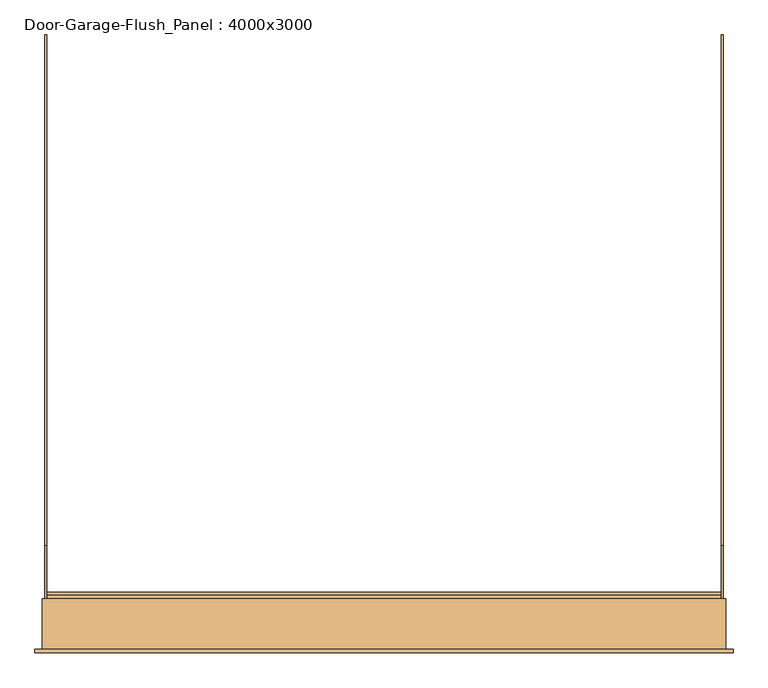
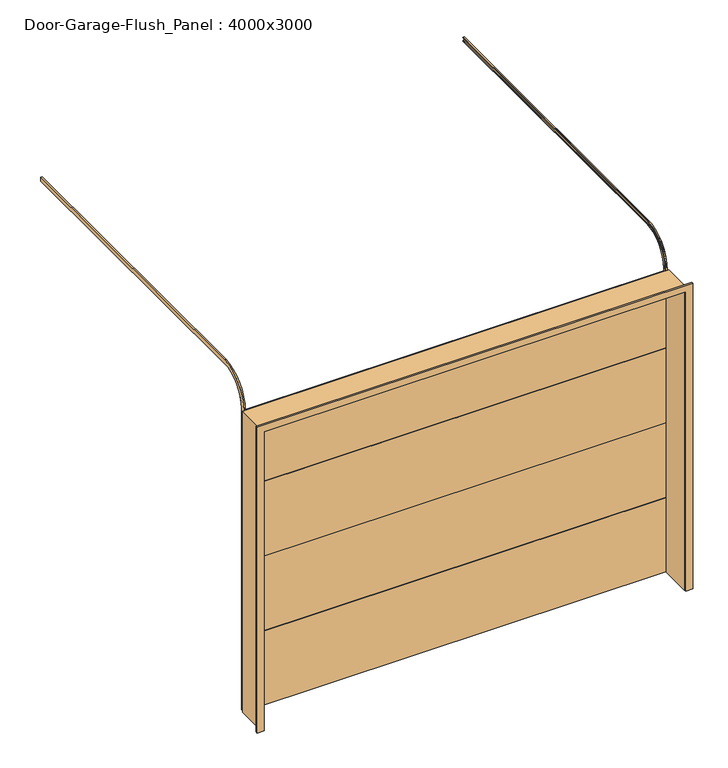
"""IFC4 building model written with IfcOpenShell, lengths in millimetres: door geometry, Door-Garage-Flush_Panel : 4000x3000."""

from ifc_helpers import new_model, si_unit, frame, origin, place, context, project, spatial, polyline, circle_curve, outline, extrude, source, transform, mapped, element, save
from ifc_brep_helpers import plane_surface, cylinder_surface, revolved_surface, advanced_brep


def door_garage_flush_panel_4000x3000_59d66c1f(model_context):
    return source(origin(), model_context, "Body", "SolidModel", [
        extrude(outline(polyline([(175.4, 3003.175), (191.275, 3003.175), (191.275, 2256.35), (169.05, 2256.35), (169.05, 2250.0), (153.175, 2250.0), (153.175, 2996.825), (175.4, 2996.825), (175.4, 3003.175)])), frame((-2000.0, 0.0, 0.0), z_axis=(1.0, 0.0, 0.0), x_axis=(0.0, 1.0, 0.0)), (0.0, 0.0, 1.0), 4000.0),
        extrude(outline(polyline([(175.4, 2253.175), (191.275, 2253.175), (191.275, 1506.35), (169.05, 1506.35), (169.05, 1500.0), (153.175, 1500.0), (153.175, 2246.825), (175.4, 2246.825), (175.4, 2253.175)])), frame((-2000.0, 0.0, 0.0), z_axis=(1.0, 0.0, 0.0), x_axis=(0.0, 1.0, 0.0)), (0.0, 0.0, 1.0), 4000.0),
        extrude(outline(polyline([(175.4, 1503.175), (191.275, 1503.175), (191.275, 756.35), (169.05, 756.35), (169.05, 750.0), (153.175, 750.0), (153.175, 1496.825), (175.4, 1496.825), (175.4, 1503.175)])), frame((-2000.0, 0.0, 0.0), z_axis=(1.0, 0.0, 0.0), x_axis=(0.0, 1.0, 0.0)), (0.0, 0.0, 1.0), 4000.0),
        extrude(outline(polyline([(175.4, 753.175), (191.275, 753.175), (191.275, 6.35), (169.05, 6.35), (169.05, 0.0), (153.175, 0.0), (153.175, 746.825), (175.4, 746.825), (175.4, 753.175)])), frame((-2000.0, 0.0, 0.0), z_axis=(1.0, 0.0, 0.0), x_axis=(0.0, 1.0, 0.0)), (0.0, 0.0, 1.0), 4000.0),
        extrude(outline(polyline([(0.0, 2025.4), (3025.4, 2025.4), (3025.4, -2025.4), (0.0, -2025.4), (0.0, -2000.0), (3000.0, -2000.0), (3000.0, 2000.0), (0.0, 2000.0), (0.0, 2025.4)])), frame((0.0, -146.825, 0.0), z_axis=(0.0, 1.0, 0.0), x_axis=(0.0, 0.0, 1.0)), (0.0, 0.0, 1.0), 300.0),
        advanced_brep(
        [(2012.7, 3496.075, 3304.8), (2000.0, 3496.075, 3304.8), (2000.0, 3496.075, 3307.975), (2009.525, 3496.075, 3307.975), (2009.525, 3496.075, 3339.725), (2000.0, 3496.075, 3339.725), (2000.0, 3496.075, 3342.9), (2012.7, 3496.075, 3342.9), (2012.7, 470.675, 3342.9), (2012.7, 153.175, 3025.4), (2012.7, 153.175, 0.0), (2012.7, 191.275, 0.0), (2012.7, 191.275, 3025.4), (2012.7, 470.675, 3304.8), (2000.0, 470.675, 3342.9), (2000.0, 470.675, 3339.725), (2000.0, 156.35, 3025.4), (2000.0, 156.35, 0.0), (2000.0, 153.175, 0.0), (2000.0, 153.175, 3025.4), (2009.525, 470.675, 3339.725), (2009.525, 470.675, 3307.975), (2009.525, 188.1, 3025.4), (2009.525, 188.1, 0.0), (2009.525, 156.35, 0.0), (2009.525, 156.35, 3025.4), (2000.0, 470.675, 3307.975), (2000.0, 470.675, 3304.8), (2000.0, 191.275, 3025.4), (2000.0, 191.275, 0.0), (2000.0, 188.1, 0.0), (2000.0, 188.1, 3025.4)],
        [
            (0, 1),
            (1, 2),
            (2, 3),
            (3, 4),
            (4, 5),
            (5, 6),
            (6, 7),
            (7, 0),
            (7, 8),
            (8, 9, circle_curve(frame((2012.7, 470.675, 3025.4), z_axis=(1.0, 0.0, 0.0), x_axis=(0.0, 0.0, 1.0)), 317.5)),
            (9, 10),
            (10, 11),
            (11, 12),
            (12, 13, circle_curve(frame((2012.7, 470.675, 3025.4), z_axis=(-1.0, 0.0, 0.0), x_axis=(0.0, 0.0, 1.0)), 279.4)),
            (13, 0),
            (6, 14),
            (14, 8),
            (5, 15),
            (15, 16, circle_curve(frame((2000.0, 470.675, 3025.4), z_axis=(1.0, 0.0, 0.0), x_axis=(0.0, 0.0, 1.0)), 314.325)),
            (16, 17),
            (17, 18),
            (18, 19),
            (19, 14, circle_curve(frame((2000.0, 470.675, 3025.4), z_axis=(-1.0, 0.0, 0.0), x_axis=(0.0, 0.0, 1.0)), 317.5)),
            (4, 20),
            (20, 15),
            (3, 21),
            (21, 22, circle_curve(frame((2009.525, 470.675, 3025.4), z_axis=(1.0, 0.0, 0.0), x_axis=(0.0, 0.0, 1.0)), 282.575)),
            (22, 23),
            (23, 24),
            (24, 25),
            (25, 20, circle_curve(frame((2009.525, 470.675, 3025.4), z_axis=(-1.0, 0.0, 0.0), x_axis=(0.0, 0.0, 1.0)), 314.325)),
            (2, 26),
            (26, 21),
            (1, 27),
            (27, 28, circle_curve(frame((2000.0, 470.675, 3025.4), z_axis=(1.0, 0.0, 0.0), x_axis=(0.0, 0.0, 1.0)), 279.4)),
            (28, 29),
            (29, 30),
            (30, 31),
            (31, 26, circle_curve(frame((2000.0, 470.675, 3025.4), z_axis=(-1.0, 0.0, 0.0), x_axis=(0.0, 0.0, 1.0)), 282.575)),
            (13, 27),
            (19, 9),
            (25, 16),
            (31, 22),
            (12, 28),
            (10, 18),
            (17, 24),
            (23, 30),
            (29, 11),
        ],
        [
            plane_surface(frame((0.0, 3496.075, 3304.8), z_axis=(0.0, 1.0, 0.0), x_axis=(1.0, 0.0, 0.0))),
            plane_surface(frame((2012.7, 3496.075, 3304.8), z_axis=(1.0, 0.0, 0.0), x_axis=(0.0, -1.0, 0.0))),
            plane_surface(frame((2012.7, 3496.075, 3342.9), z_axis=(0.0, 0.0, 1.0), x_axis=(0.0, -1.0, 0.0))),
            plane_surface(frame((2000.0, 3496.075, 3342.9), z_axis=(-1.0, 0.0, 0.0), x_axis=(0.0, -1.0, 0.0))),
            plane_surface(frame((2000.0, 3496.075, 3339.725), z_axis=(0.0, 0.0, -1.0), x_axis=(0.0, -1.0, 0.0))),
            plane_surface(frame((2009.525, 3496.075, 3339.725), z_axis=(-1.0, 0.0, 0.0), x_axis=(0.0, -1.0, 0.0))),
            plane_surface(frame((2009.525, 3496.075, 3307.975), z_axis=(0.0, 0.0, 1.0), x_axis=(0.0, -1.0, 0.0))),
            plane_surface(frame((2000.0, 3496.075, 3307.975), z_axis=(-1.0, 0.0, 0.0), x_axis=(0.0, -1.0, 0.0))),
            plane_surface(frame((2000.0, 3496.075, 3304.8), z_axis=(0.0, 0.0, -1.0), x_axis=(0.0, -1.0, 0.0))),
            cylinder_surface(frame((0.0, 470.675, 3025.4), z_axis=(-1.0, 0.0, 0.0), x_axis=(0.0, 0.0, 1.0)), 317.5),
            revolved_surface(polyline([(2000.0, 470.675, 3339.725), (2009.525, 470.675, 3339.725)]), (0.0, 470.675, 3025.4), (-1.0, 0.0, 0.0)),
            cylinder_surface(frame((0.0, 470.675, 3025.4), z_axis=(-1.0, 0.0, 0.0), x_axis=(0.0, 0.0, 1.0)), 282.575),
            revolved_surface(polyline([(2000.0, 470.675, 3304.8), (2012.7, 470.675, 3304.8)]), (0.0, 470.675, 3025.4), (-1.0, 0.0, 0.0)),
            plane_surface(frame((0.0, 191.275, 0.0), z_axis=(0.0, 0.0, -1.0), x_axis=(1.0, 0.0, 0.0))),
            plane_surface(frame((2012.7, 153.175, 3025.4), z_axis=(0.0, -1.0, 0.0), x_axis=(0.0, 0.0, -1.0))),
            plane_surface(frame((2000.0, 156.35, 3025.4), z_axis=(0.0, 1.0, 0.0), x_axis=(0.0, 0.0, -1.0))),
            plane_surface(frame((2009.525, 188.1, 3025.4), z_axis=(0.0, -1.0, 0.0), x_axis=(0.0, 0.0, -1.0))),
            plane_surface(frame((2000.0, 191.275, 3025.4), z_axis=(0.0, 1.0, 0.0), x_axis=(0.0, 0.0, -1.0))),
        ],
        [
            (0, [[1, 2, 3, 4, 5, 6, 7, 8]]),
            (1, [[9, 10, 11, 12, 13, 14, 15, -8]]),
            (2, [[16, 17, -9, -7]]),
            (3, [[18, 19, 20, 21, 22, 23, -16, -6]]),
            (4, [[24, 25, -18, -5]]),
            (5, [[26, 27, 28, 29, 30, 31, -24, -4]]),
            (6, [[32, 33, -26, -3]]),
            (7, [[34, 35, 36, 37, 38, 39, -32, -2]]),
            (8, [[-15, 40, -34, -1]]),
            (9, [[41, -10, -17, -23]]),
            (10, [[42, -19, -25, -31]]),
            (11, [[43, -27, -33, -39]]),
            (12, [[44, -35, -40, -14]]),
            (13, [[-12, 45, -21, 46, -29, 47, -37, 48]]),
            (14, [[-22, -45, -11, -41]]),
            (15, [[-30, -46, -20, -42]]),
            (16, [[-38, -47, -28, -43]]),
            (17, [[-13, -48, -36, -44]]),
        ],
    ),
        advanced_brep(
        [(-2012.7, 3496.075, 3304.8), (-2012.7, 3496.075, 3342.9), (-2000.0, 3496.075, 3342.9), (-2000.0, 3496.075, 3339.725), (-2009.525, 3496.075, 3339.725), (-2009.525, 3496.075, 3307.975), (-2000.0, 3496.075, 3307.975), (-2000.0, 3496.075, 3304.8), (-2000.0, 470.675, 3304.8), (-2012.7, 470.675, 3304.8), (-2000.0, 470.675, 3307.975), (-2000.0, 188.1, 3025.4), (-2000.0, 188.1, 0.0), (-2000.0, 191.275, 0.0), (-2000.0, 191.275, 3025.4), (-2009.525, 470.675, 3307.975), (-2009.525, 470.675, 3339.725), (-2009.525, 156.35, 3025.4), (-2009.525, 156.35, 0.0), (-2009.525, 188.1, 0.0), (-2009.525, 188.1, 3025.4), (-2000.0, 470.675, 3339.725), (-2000.0, 470.675, 3342.9), (-2000.0, 153.175, 3025.4), (-2000.0, 153.175, 0.0), (-2000.0, 156.35, 0.0), (-2000.0, 156.35, 3025.4), (-2012.7, 470.675, 3342.9), (-2012.7, 191.275, 3025.4), (-2012.7, 191.275, 0.0), (-2012.7, 153.175, 0.0), (-2012.7, 153.175, 3025.4)],
        [
            (0, 1),
            (1, 2),
            (2, 3),
            (3, 4),
            (4, 5),
            (5, 6),
            (6, 7),
            (7, 0),
            (7, 8),
            (8, 9),
            (9, 0),
            (6, 10),
            (10, 11, circle_curve(frame((-2000.0, 470.675, 3025.4), z_axis=(1.0, 0.0, 0.0), x_axis=(0.0, 0.0, 1.0)), 282.575)),
            (11, 12),
            (12, 13),
            (13, 14),
            (14, 8, circle_curve(frame((-2000.0, 470.675, 3025.4), z_axis=(-1.0, 0.0, 0.0), x_axis=(0.0, 0.0, 1.0)), 279.4)),
            (5, 15),
            (15, 10),
            (4, 16),
            (16, 17, circle_curve(frame((-2009.525, 470.675, 3025.4), z_axis=(1.0, 0.0, 0.0), x_axis=(0.0, 0.0, 1.0)), 314.325)),
            (17, 18),
            (18, 19),
            (19, 20),
            (20, 15, circle_curve(frame((-2009.525, 470.675, 3025.4), z_axis=(-1.0, 0.0, 0.0), x_axis=(0.0, 0.0, 1.0)), 282.575)),
            (3, 21),
            (21, 16),
            (2, 22),
            (22, 23, circle_curve(frame((-2000.0, 470.675, 3025.4), z_axis=(1.0, 0.0, 0.0), x_axis=(0.0, 0.0, 1.0)), 317.5)),
            (23, 24),
            (24, 25),
            (25, 26),
            (26, 21, circle_curve(frame((-2000.0, 470.675, 3025.4), z_axis=(-1.0, 0.0, 0.0), x_axis=(0.0, 0.0, 1.0)), 314.325)),
            (1, 27),
            (27, 22),
            (9, 28, circle_curve(frame((-2012.7, 470.675, 3025.4), z_axis=(1.0, 0.0, 0.0), x_axis=(0.0, 0.0, 1.0)), 279.4)),
            (28, 29),
            (29, 30),
            (30, 31),
            (31, 27, circle_curve(frame((-2012.7, 470.675, 3025.4), z_axis=(-1.0, 0.0, 0.0), x_axis=(0.0, 0.0, 1.0)), 317.5)),
            (14, 28),
            (20, 11),
            (26, 17),
            (31, 23),
            (29, 13),
            (12, 19),
            (18, 25),
            (24, 30),
        ],
        [
            plane_surface(frame((0.0, 3496.075, 3304.8), z_axis=(0.0, 1.0, 0.0), x_axis=(1.0, 0.0, 0.0))),
            plane_surface(frame((-2012.7, 3496.075, 3304.8), z_axis=(0.0, 0.0, -1.0), x_axis=(0.0, -1.0, 0.0))),
            plane_surface(frame((-2000.0, 3496.075, 3304.8), z_axis=(1.0, 0.0, 0.0), x_axis=(0.0, -1.0, 0.0))),
            plane_surface(frame((-2000.0, 3496.075, 3307.975), z_axis=(0.0, 0.0, 1.0), x_axis=(0.0, -1.0, 0.0))),
            plane_surface(frame((-2009.525, 3496.075, 3307.975), z_axis=(1.0, 0.0, 0.0), x_axis=(0.0, -1.0, 0.0))),
            plane_surface(frame((-2009.525, 3496.075, 3339.725), z_axis=(0.0, 0.0, -1.0), x_axis=(0.0, -1.0, 0.0))),
            plane_surface(frame((-2000.0, 3496.075, 3339.725), z_axis=(1.0, 0.0, 0.0), x_axis=(0.0, -1.0, 0.0))),
            plane_surface(frame((-2000.0, 3496.075, 3342.9), z_axis=(0.0, 0.0, 1.0), x_axis=(0.0, -1.0, 0.0))),
            plane_surface(frame((-2012.7, 3496.075, 3342.9), z_axis=(-1.0, 0.0, 0.0), x_axis=(0.0, -1.0, 0.0))),
            revolved_surface(polyline([(-2012.7, 470.675, 3304.8), (-2000.0, 470.675, 3304.8)]), (0.0, 470.675, 3025.4), (-1.0, 0.0, 0.0)),
            cylinder_surface(frame((0.0, 470.675, 3025.4), z_axis=(-1.0, 0.0, 0.0), x_axis=(0.0, 0.0, 1.0)), 282.575),
            revolved_surface(polyline([(-2009.525, 470.675, 3339.725), (-2000.0, 470.675, 3339.725)]), (0.0, 470.675, 3025.4), (-1.0, 0.0, 0.0)),
            cylinder_surface(frame((0.0, 470.675, 3025.4), z_axis=(-1.0, 0.0, 0.0), x_axis=(0.0, 0.0, 1.0)), 317.5),
            plane_surface(frame((0.0, 191.275, 0.0), z_axis=(0.0, 0.0, -1.0), x_axis=(1.0, 0.0, 0.0))),
            plane_surface(frame((-2012.7, 191.275, 3025.4), z_axis=(0.0, 1.0, 0.0), x_axis=(0.0, 0.0, -1.0))),
            plane_surface(frame((-2000.0, 188.1, 3025.4), z_axis=(0.0, -1.0, 0.0), x_axis=(0.0, 0.0, -1.0))),
            plane_surface(frame((-2009.525, 156.35, 3025.4), z_axis=(0.0, 1.0, 0.0), x_axis=(0.0, 0.0, -1.0))),
            plane_surface(frame((-2000.0, 153.175, 3025.4), z_axis=(0.0, -1.0, 0.0), x_axis=(0.0, 0.0, -1.0))),
        ],
        [
            (0, [[1, 2, 3, 4, 5, 6, 7, 8]]),
            (1, [[9, 10, 11, -8]]),
            (2, [[12, 13, 14, 15, 16, 17, -9, -7]]),
            (3, [[18, 19, -12, -6]]),
            (4, [[20, 21, 22, 23, 24, 25, -18, -5]]),
            (5, [[26, 27, -20, -4]]),
            (6, [[28, 29, 30, 31, 32, 33, -26, -3]]),
            (7, [[34, 35, -28, -2]]),
            (8, [[-11, 36, 37, 38, 39, 40, -34, -1]]),
            (9, [[41, -36, -10, -17]]),
            (10, [[42, -13, -19, -25]]),
            (11, [[43, -21, -27, -33]]),
            (12, [[44, -29, -35, -40]]),
            (13, [[45, -15, 46, -23, 47, -31, 48, -38]]),
            (14, [[-16, -45, -37, -41]]),
            (15, [[-24, -46, -14, -42]]),
            (16, [[-32, -47, -22, -43]]),
            (17, [[-39, -48, -30, -44]]),
        ],
    ),
        extrude(outline(polyline([(0.0, 2069.85), (3069.85, 2069.85), (3069.85, -2069.85), (0.0, -2069.85), (0.0, -2006.35), (3006.35, -2006.35), (3006.35, 2006.35), (0.0, 2006.35), (0.0, 2069.85)])), frame((0.0, -165.875, 0.0), z_axis=(0.0, 1.0, 0.0), x_axis=(0.0, 0.0, 1.0)), (0.0, 0.0, 1.0), 19.05),
    ])


if __name__ == "__main__":
    model = new_model("IFC4")
    model_context = context("Model", 3, world=origin())
    ifc_project = project(units=[si_unit("LENGTHUNIT", "METRE", prefix="MILLI")], contexts=[model_context])
    site = spatial("IfcSite", under=ifc_project)
    building = spatial("IfcBuilding", under=site)
    placement = place(None, origin())
    door_garage_flush_panel_4000x3000_shape = door_garage_flush_panel_4000x3000_59d66c1f(model_context)
    element("IfcDoor", 1, ObjectType="Door-Garage-Flush_Panel : 4000x3000", at=placement, inside=building, context=model_context, shape_type="MappedRepresentation", body=[
        mapped(door_garage_flush_panel_4000x3000_shape, transform((0.0, 0.0, 0.0), x_axis=(1.0, 0.0, 0.0), y_axis=(0.0, 1.0, 0.0), z_axis=(0.0, 0.0, 1.0))),
    ])
    save(model, "model.ifc")

# Revit data of these elements
# Type "Door-Garage-Flush_Panel : 4000x3000"
#   Type Mark = "41"
#   Assembly Code = "B2030400"
#   Analytic Construction = "Wooden"
#   Thickness = 38.1 mm
#   Thermal Resistance (R) = 0.455703 (m²·K)/W
#   Rough Width = 4050.8 mm
#   Rough Height = 3025.4 mm
#   Panel Height = 750 mm
#   Height = 3000 mm
#   Width = 4000 mm
#   Heat Transfer Coefficient (U) = 2.19465 W/(m²·K)
#   Function = 1
#   Exterior Trim [instance default] = yes
#   Trim Material = Cherry
#   Panel Material = Cherry
#   Frame Material = Cherry
#   Visual Light Transmittance = 0
#   Solar Heat Gain Coefficient = 0
#   Wall Closure = (empty or 0)
# Element 1 (IfcDoor, "Door-Garage-Flush_Panel : 4000x3000")
#   Materials on its faces: "Cherry"
# Materials
#   "Cherry": class "Wood", colour RGB 226 177 128, transparency 0, Description = "Prunus Serotina", Cost = 0
